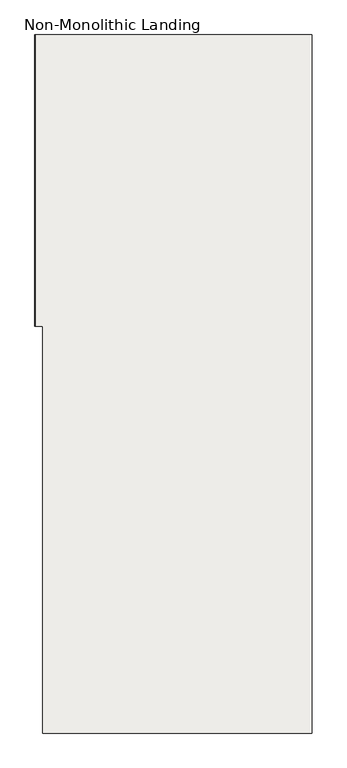
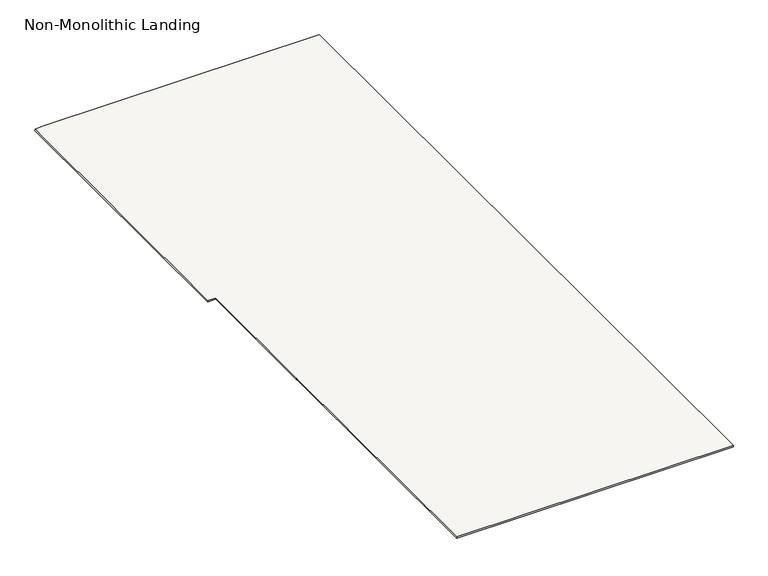
"""IFC4 building model written with IfcOpenShell, lengths in millimetres: slab geometry, Non-Monolithic Landing."""

from ifc_helpers import new_model, si_unit, origin, place, context, project, spatial, faceted_brep, source, transform, mapped, element, save


def non_monolithic_landing_c698f8d3(model_context):
    return source(origin(), model_context, "Body", "Brep", [
        faceted_brep([(16318.9400908, 13220.4345331, 14176.4705882), (16318.0900908, 13220.4345331, 14170.4705882), (16318.0900908, 12030.4345331, 14170.4705882), (16318.9400908, 12030.4345331, 14176.4705882), (16350.0, 10370.4345331, 14176.4705882), (17450.0, 10370.4345331, 14176.4705882), (17450.0, 13220.4345331, 14176.4705882), (16350.0, 13220.4345331, 14176.4705882), (16350.0, 12030.4345331, 14176.4705882), (16350.0, 11470.4345331, 14176.4705882), (17450.0, 13220.4345331, 14170.4705882), (17450.0, 10370.4345331, 14170.4705882), (16350.85, 10370.4345331, 14170.4705882), (16350.85, 11470.4345331, 14170.4705882), (16350.0, 11470.4345331, 14170.4705882), (16350.0, 12030.4345331, 14170.4705882), (16350.0, 13220.4345331, 14170.4705882)], [[[0, 1, 2, 3]], [[4, 5, 6, 7, 0, 3, 8, 9]], [[10, 11, 12, 13, 14, 15, 2, 1, 16]], [[9, 8, 15, 14]], [[0, 7, 16, 1]], [[7, 6, 10, 16]], [[6, 5, 11, 10]], [[5, 4, 12, 11]], [[13, 9, 14]], [[9, 13, 12, 4]], [[8, 3, 2, 15]]]),
    ])


if __name__ == "__main__":
    model = new_model("IFC4")
    model_context = context("Model", 3, world=origin())
    ifc_project = project(units=[si_unit("LENGTHUNIT", "METRE", prefix="MILLI")], contexts=[model_context])
    site = spatial("IfcSite", under=ifc_project)
    building = spatial("IfcBuilding", under=site)
    placement = place(None, origin())
    non_monolithic_landing_shape = non_monolithic_landing_c698f8d3(model_context)
    element("IfcSlab", 1, ObjectType="Non-Monolithic Landing", at=placement, inside=building, context=model_context, shape_type="MappedRepresentation", body=[
        mapped(non_monolithic_landing_shape, transform((0.0, 0.0, 0.0), x_axis=(1.0, 0.0, 0.0), y_axis=(0.0, 1.0, 0.0), z_axis=(0.0, 0.0, 1.0))),
    ])
    save(model, "model.ifc")

# Revit data of these elements
# Element 1 (IfcSlab, "Non-Monolithic Landing")
#   Materials on its faces: "Steel, Paint Finish, Dark Gray"
# Materials
#   "Steel, Paint Finish, Dark Gray": class "Metal", colour RGB 89 89 89, transparency 0, Description = "Steel, paint finish, dark gray, glossy", Cost = 0
